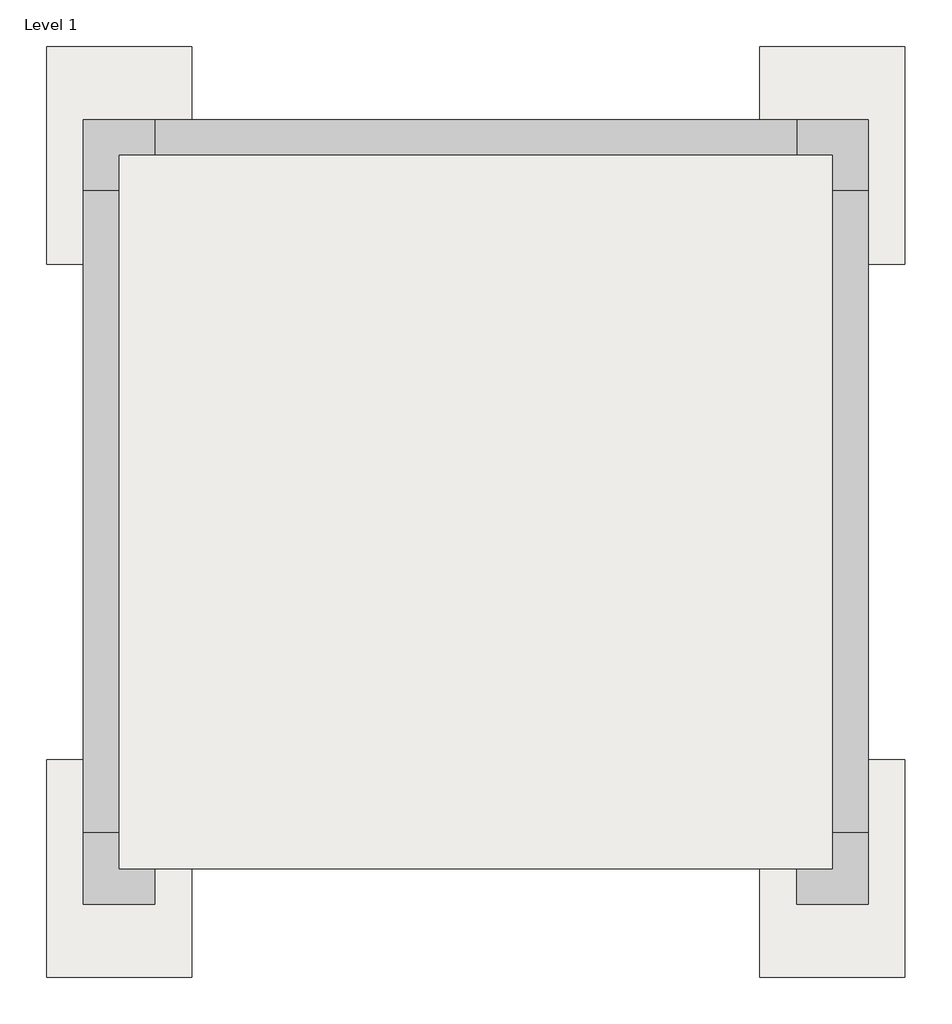
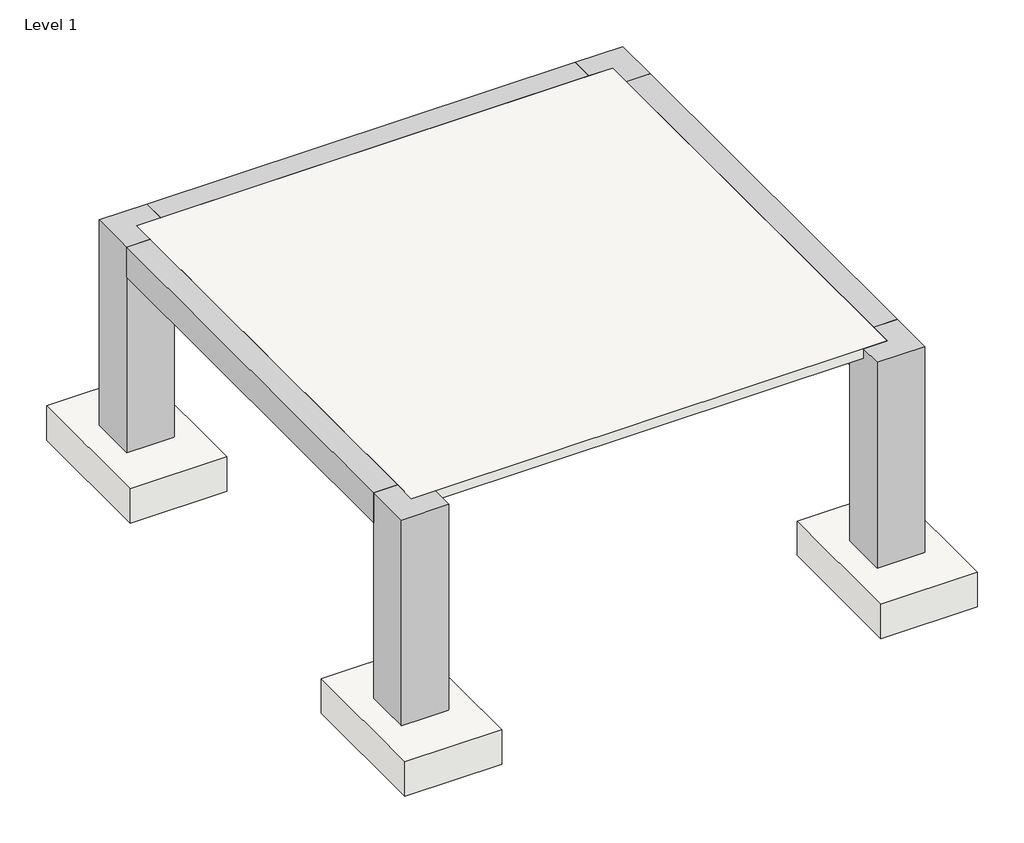
# One storey: 5 slabs, 4 columns, 3 beams.
"""IFC4 building model written with IfcOpenShell, lengths in millimetres."""

import ifcopenshell
import ifcopenshell.guid

model = None  # the IFC model being written
_history = None  # IfcOwnerHistory: only IFC2X3 demands one
_inside = {}  # id of a spatial element -> (the spatial element, [elements in it])
_under = {}  # id of a project, library or spatial element -> (it, [spatial elements below it])
_declared = {}  # id of a project -> (the project, [libraries it declares])
_typed = {}  # id of a type object -> (the type object, [elements of that type])
_made_of = {}  # id of a material, layer set ... -> (it, [elements and type objects made of it])


def new_model(schema):
    """Start an empty IFC model of exactly this schema.

    Asked for "IFC4X3", IfcOpenShell would pick the latest addendum, in which some entities
    have other attributes; the version numbers below select the first issue.
    IFC2X3 requires an IfcOwnerHistory on every rooted entity: one is made here for all.
    """
    global model, _history
    if schema == "IFC4X3":
        model = ifcopenshell.file(schema_version=(4, 3, 0, 0))
    else:
        model = ifcopenshell.file(schema=schema)
    _inside.clear()
    _under.clear()
    _declared.clear()
    _typed.clear()
    _made_of.clear()
    _history = None
    if model.schema == "IFC2X3":
        org = make("IfcOrganization", Name="unknown")
        user = make(
            "IfcPersonAndOrganization",
            ThePerson=make("IfcPerson", FamilyName="unknown"),
            TheOrganization=org,
        )
        app = make(
            "IfcApplication",
            ApplicationDeveloper=org,
            Version="unknown",
            ApplicationFullName="unknown",
            ApplicationIdentifier="unknown",
        )
        _history = make(
            "IfcOwnerHistory",
            OwningUser=user,
            OwningApplication=app,
            ChangeAction="ADDED",
            CreationDate=0,
        )
    return model


def make(cls, **values):
    """One entity of the class cls with the attributes given. An attribute that is None is left unset."""
    return model.create_entity(
        cls, **{name: value for name, value in values.items() if value is not None}
    )


def rooted(cls, **values):
    """An entity with a GlobalId (a new one), such as an element, a storey or a relation."""
    return make(cls, GlobalId=ifcopenshell.guid.new(), OwnerHistory=_history, **values)


def si_unit(unit_type, name, prefix=None):
    """IfcSIUnit, for example si_unit("LENGTHUNIT", "METRE", prefix="MILLI")."""
    return make("IfcSIUnit", UnitType=unit_type, Prefix=prefix, Name=name)


def assignment(units):
    """IfcUnitAssignment: the units of a project."""
    return None if units is None else make("IfcUnitAssignment", Units=units)


def point(xyz):
    """IfcCartesianPoint."""
    return None if xyz is None else make("IfcCartesianPoint", Coordinates=xyz)


def direction(xyz):
    """IfcDirection."""
    return None if xyz is None else make("IfcDirection", DirectionRatios=xyz)


def frame(location, z_axis=None, x_axis=None):
    """IfcAxis2Placement3D, a coordinate frame: its origin and axes. An axis left out is left unset."""
    return make(
        "IfcAxis2Placement3D",
        Location=point(location),
        Axis=direction(z_axis),
        RefDirection=direction(x_axis),
    )


def origin():
    """The frame at (0, 0, 0) with its axes left unset."""
    return frame((0.0, 0.0, 0.0))


def place(relative_to, where):
    """IfcLocalPlacement: puts the frame where relative to a parent placement (None: the world)."""
    return make(
        "IfcLocalPlacement", PlacementRelTo=relative_to, RelativePlacement=where
    )


def context(
    kind, dimensions, precision=None, world=None, true_north=None, identifier=None
):
    """IfcGeometricRepresentationContext, for example the 3D "Model" context."""
    return make(
        "IfcGeometricRepresentationContext",
        ContextIdentifier=identifier,
        ContextType=kind,
        CoordinateSpaceDimension=dimensions,
        Precision=precision,
        WorldCoordinateSystem=world,
        TrueNorth=true_north,
    )


def project(units=None, contexts=None):
    """IfcProject with its units and contexts."""
    return rooted(
        "IfcProject",
        Name="project",
        RepresentationContexts=contexts,
        UnitsInContext=assignment(units),
    )


def spatial(cls, under=None, at=None, **own):
    """A site, building, storey or space (cls), placed at a placement, below another one or the project."""
    s = rooted(cls, ObjectPlacement=at, **own)
    if under is not None:
        _under.setdefault(under.id(), (under, []))[1].append(s)
    return s


def polyline(points):
    """IfcPolyline through the points."""
    return make("IfcPolyline", Points=[point(p) for p in points])


def outline(outer, holes=None, kind="AREA"):
    """IfcArbitraryClosedProfileDef: a profile drawn as a closed curve; with holes, ...WithVoids."""
    if holes is None:
        return make("IfcArbitraryClosedProfileDef", ProfileType=kind, OuterCurve=outer)
    return make(
        "IfcArbitraryProfileDefWithVoids",
        ProfileType=kind,
        OuterCurve=outer,
        InnerCurves=holes,
    )


def extrude(swept, where, along, depth):
    """IfcExtrudedAreaSolid: the profile swept, set in the frame where, extruded along a direction by depth."""
    return make(
        "IfcExtrudedAreaSolid",
        SweptArea=swept,
        Position=where,
        ExtrudedDirection=direction(along),
        Depth=depth,
    )


def faces_of(points, faces, orient=None, outer=None):
    """IfcFace entities. A face is a list of loops; a loop is a list of indices into points, from 0.

    orient and outer hold one flag for each loop. By default every Orientation is true, the
    first loop of a face is its IfcFaceOuterBound and the others are IfcFaceBound.
    """
    made = []
    for i, loops in enumerate(faces):
        bounds = []
        for j, loop in enumerate(loops):
            is_outer = j == 0 if outer is None else outer[i][j]
            bounds.append(
                make(
                    "IfcFaceOuterBound" if is_outer else "IfcFaceBound",
                    Bound=make("IfcPolyLoop", Polygon=[points[k] for k in loop]),
                    Orientation=True if orient is None else orient[i][j],
                )
            )
        made.append(make("IfcFace", Bounds=bounds))
    return made


def faceted_brep(points, faces, orient=None, outer=None, voids=None):
    """IfcFacetedBrep: a solid bounded by flat faces; with voids (closed shells), ...WithVoids."""
    shared = [point(p) for p in points]
    hull = make("IfcClosedShell", CfsFaces=faces_of(shared, faces, orient, outer))
    if voids is None:
        return make("IfcFacetedBrep", Outer=hull)
    return make(
        "IfcFacetedBrepWithVoids",
        Outer=hull,
        Voids=[
            make(cls, CfsFaces=faces_of(shared, fs, o, b)) for cls, fs, o, b in voids
        ],
    )


def shape(context_of_items, identifier, shape_type, items):
    """IfcShapeRepresentation: the items that make up one representation, for example the "Body"."""
    return make(
        "IfcShapeRepresentation",
        ContextOfItems=context_of_items,
        RepresentationIdentifier=identifier,
        RepresentationType=shape_type,
        Items=items,
    )


def source(mapping_origin, context_of_items, identifier, shape_type, items):
    """IfcRepresentationMap: a shape defined once, which mapped items show again and again."""
    return make(
        "IfcRepresentationMap",
        MappingOrigin=mapping_origin,
        MappedRepresentation=shape(context_of_items, identifier, shape_type, items),
    )


def transform(
    local_origin,
    x_axis=None,
    y_axis=None,
    z_axis=None,
    scale=None,
    scale2=None,
    scale3=None,
    uniform=True,
):
    """IfcCartesianTransformationOperator3D, or its non-uniform kind. x_axis, y_axis, z_axis: its Axis1, 2, 3."""
    if uniform:
        return make(
            "IfcCartesianTransformationOperator3D",
            Axis1=direction(x_axis),
            Axis2=direction(y_axis),
            LocalOrigin=point(local_origin),
            Scale=scale,
            Axis3=direction(z_axis),
        )
    return make(
        "IfcCartesianTransformationOperator3DnonUniform",
        Axis1=direction(x_axis),
        Axis2=direction(y_axis),
        LocalOrigin=point(local_origin),
        Scale=scale,
        Axis3=direction(z_axis),
        Scale2=scale2,
        Scale3=scale3,
    )


def mapped(mapping_source, mapping_target):
    """IfcMappedItem: shows the shape of a source again, moved by a transform."""
    return make(
        "IfcMappedItem", MappingSource=mapping_source, MappingTarget=mapping_target
    )


def made_of(thing, what):
    """Note that an element or type object is made of a material, layer set ...; save() writes the relation."""
    if what is not None:
        _made_of.setdefault(what.id(), (what, []))[1].append(thing)
    return thing


def element(
    cls,
    number,
    at=None,
    inside=None,
    cuts=None,
    type_object=None,
    material=None,
    context=None,
    identifier="Body",
    shape_type=None,
    held_by="IfcProductDefinitionShape",
    body=None,
    shapes=None,
    **own,
):
    """One element of the class cls, such as IfcWall. Its Tag is "e" and its number.

    at: its placement. inside: the storey or other place that contains it. cuts: it is an
    opening in that element (IfcRelVoidsElement). A single representation is given by context,
    identifier, shape_type and body (its items); several are given by shapes. held_by: the class
    of the entity that holds the representations. save() writes the other relations.
    """
    e = rooted(cls, Tag="e%d" % number, ObjectPlacement=at, **own)
    if body is not None:
        shapes = [shape(context, identifier, shape_type, body)]
    if shapes is not None:
        e.Representation = make(held_by, Representations=shapes)
    if inside is not None:
        _inside.setdefault(inside.id(), (inside, []))[1].append(e)
    if cuts is not None:
        rooted(
            "IfcRelVoidsElement", RelatingBuildingElement=cuts, RelatedOpeningElement=e
        )
    if type_object is not None:
        _typed.setdefault(type_object.id(), (type_object, []))[1].append(e)
    return made_of(e, material)


def aggregate(whole, parts):
    """IfcRelAggregates: a whole, such as a stair, and the parts it consists of."""
    return rooted("IfcRelAggregates", RelatingObject=whole, RelatedObjects=parts)


def save(model, path):
    """Write the relations noted so far, then the file.

    IfcRelAggregates (storeys below a building ...), IfcRelContainedInSpatialStructure (elements
    in a storey), IfcRelDefinesByType, IfcRelAssociatesMaterial and IfcRelDeclares: one each for
    every whole, place, type object, material and project.
    """
    for whole, parts in _under.values():
        aggregate(whole, parts)
    for where, things in _inside.values():
        rooted(
            "IfcRelContainedInSpatialStructure",
            RelatedElements=things,
            RelatingStructure=where,
        )
    for kind, things in _typed.values():
        rooted("IfcRelDefinesByType", RelatedObjects=things, RelatingType=kind)
    for what, things in _made_of.values():
        rooted("IfcRelAssociatesMaterial", RelatedObjects=things, RelatingMaterial=what)
    for by, libraries in _declared.values():
        rooted("IfcRelDeclares", RelatingContext=by, RelatedDefinitions=libraries)
    model.write(path)


def slab_5ba74754(model_context):
    return source(origin(), model_context, "Body", "SweptSolid", [
        extrude(outline(polyline([(609.6, 914.4), (609.6, -914.4), (-609.6, -914.4), (-609.6, 914.4), (609.6, 914.4)])), frame((0.0, 0.0, -457.2), z_axis=(0.0, 0.0, 1.0), x_axis=(1.0, 0.0, 0.0)), (0.0, 0.0, 1.0), 457.2),
    ])


model = new_model("IFC4")

# Units and contexts
model_context = context("Model", 3, world=origin())
ifc_project = project(units=[si_unit("LENGTHUNIT", "METRE", prefix="MILLI")], contexts=[model_context])

# Site, building, storey
site = spatial("IfcSite", under=ifc_project)
building = spatial("IfcBuilding", under=site)
storey = spatial("IfcBuildingStorey", under=building, Name="Level 1", Elevation=0.0)

# Beams
placement = place(None, origin())
element("IfcBeam", 1, ObjectType="Concrete-Rectangular Beam : 60 x 40", at=placement, inside=storey, context=model_context, shape_type="SweptSolid", body=[
    extrude(outline(polyline([(2988.1334536, -400.0), (2388.1334536, -400.0), (2388.1334536, -127.0), (2688.1334536, -127.0), (2688.1334536, 0.0), (2988.1334536, 0.0), (2988.1334536, -400.0)])), frame((-17170.3561079, 0.0, 0.0), z_axis=(1.0, 0.0, 0.0), x_axis=(0.0, 1.0, 0.0)), (0.0, 0.0, 1.0), 5400.0),
])
element("IfcBeam", 2, ObjectType="Concrete-Rectangular Beam : 60 x 40", at=placement, inside=storey, context=model_context, shape_type="SweptSolid", body=[
    extrude(outline(polyline([(0.0, -17770.3561079), (-400.0, -17770.3561079), (-400.0, -17170.3561079), (-127.0, -17170.3561079), (-127.0, -17470.3561079), (0.0, -17470.3561079), (0.0, -17770.3561079)])), frame((0.0, -3011.8665464, 0.0), z_axis=(0.0, 1.0, 0.0), x_axis=(0.0, 0.0, 1.0)), (0.0, 0.0, 1.0), 5400.0),
])
element("IfcBeam", 3, ObjectType="Concrete-Rectangular Beam : 60 x 40", at=placement, inside=storey, context=model_context, shape_type="SweptSolid", body=[
    extrude(outline(polyline([(-400.0, -11770.3561079), (-400.0, -11170.3561079), (0.0, -11170.3561079), (0.0, -11470.3561079), (-127.0, -11470.3561079), (-127.0, -11770.3561079), (-400.0, -11770.3561079)])), frame((0.0, -3011.8665464, 0.0), z_axis=(0.0, 1.0, 0.0), x_axis=(0.0, 0.0, 1.0)), (0.0, 0.0, 1.0), 5400.0),
])

# Columns
element("IfcColumn", 4, ObjectType="Concrete-Rectangular-Column : 60 x 60", at=placement, inside=storey, context=model_context, shape_type="Brep", body=[
    faceted_brep([(-17170.3561079, 2988.1334536, -2743.2), (-17170.3561079, 2388.1334536, -2743.2), (-17770.3561079, 2388.1334536, -2743.2), (-17770.3561079, 2988.1334536, -2743.2), (-17170.3561079, 2988.1334536, 0.0), (-17170.3561079, 2688.1334536, 0.0), (-17170.3561079, 2688.1334536, -127.0), (-17170.3561079, 2388.1334536, -127.0), (-17470.3561079, 2388.1334536, -127.0), (-17470.3561079, 2388.1334536, 0.0), (-17770.3561079, 2388.1334536, 0.0), (-17770.3561079, 2988.1334536, 0.0), (-17470.3561079, 2688.1334536, 0.0), (-17470.3561079, 2688.1334536, -127.0)], [[[0, 1, 2, 3]], [[1, 0, 4, 5, 6, 7]], [[2, 1, 7, 8, 9, 10]], [[3, 2, 10, 11]], [[0, 3, 11, 4]], [[11, 10, 9, 12, 5, 4]], [[6, 13, 8, 7]], [[13, 12, 9, 8]], [[12, 13, 6, 5]]]),
])
element("IfcColumn", 5, ObjectType="Concrete-Rectangular-Column : 60 x 60", at=placement, inside=storey, context=model_context, shape_type="Brep", body=[
    faceted_brep([(-11170.3561079, 2988.1334536, -2743.2), (-11170.3561079, 2388.1334536, -2743.2), (-11770.3561079, 2388.1334536, -2743.2), (-11770.3561079, 2988.1334536, -2743.2), (-11170.3561079, 2988.1334536, 0.0), (-11170.3561079, 2388.1334536, 0.0), (-11470.3561079, 2388.1334536, 0.0), (-11470.3561079, 2388.1334536, -127.0), (-11770.3561079, 2388.1334536, -127.0), (-11770.3561079, 2688.1334536, -127.0), (-11770.3561079, 2688.1334536, 0.0), (-11770.3561079, 2988.1334536, 0.0), (-11470.3561079, 2688.1334536, 0.0), (-11470.3561079, 2688.1334536, -127.0)], [[[0, 1, 2, 3]], [[1, 0, 4, 5]], [[2, 1, 5, 6, 7, 8]], [[3, 2, 8, 9, 10, 11]], [[0, 3, 11, 4]], [[5, 4, 11, 10, 12, 6]], [[7, 13, 9, 8]], [[13, 12, 10, 9]], [[12, 13, 7, 6]]]),
])
element("IfcColumn", 6, ObjectType="Concrete-Rectangular-Column : 60 x 60", at=placement, inside=storey, context=model_context, shape_type="Brep", body=[
    faceted_brep([(-11170.3561079, -3011.8665464, -2743.2), (-11170.3561079, -3611.8665464, -2743.2), (-11770.3561079, -3611.8665464, -2743.2), (-11770.3561079, -3011.8665464, -2743.2), (-11170.3561079, -3011.8665464, 0.0), (-11170.3561079, -3611.8665464, 0.0), (-11770.3561079, -3611.8665464, 0.0), (-11770.3561079, -3311.8665464, 0.0), (-11770.3561079, -3311.8665464, -127.0), (-11770.3561079, -3011.8665464, -127.0), (-11470.3561079, -3011.8665464, -127.0), (-11470.3561079, -3011.8665464, 0.0), (-11470.3561079, -3311.8665464, 0.0), (-11470.3561079, -3311.8665464, -127.0)], [[[0, 1, 2, 3]], [[1, 0, 4, 5]], [[2, 1, 5, 6]], [[3, 2, 6, 7, 8, 9]], [[0, 3, 9, 10, 11, 4]], [[5, 4, 11, 12, 7, 6]], [[8, 13, 10, 9]], [[13, 12, 11, 10]], [[12, 13, 8, 7]]]),
])
element("IfcColumn", 7, ObjectType="Concrete-Rectangular-Column : 60 x 60", at=placement, inside=storey, context=model_context, shape_type="Brep", body=[
    faceted_brep([(-17170.3561079, -3011.8665464, -2743.2), (-17170.3561079, -3611.8665464, -2743.2), (-17770.3561079, -3611.8665464, -2743.2), (-17770.3561079, -3011.8665464, -2743.2), (-17170.3561079, -3011.8665464, -127.0), (-17170.3561079, -3311.8665464, -127.0), (-17170.3561079, -3311.8665464, 0.0), (-17170.3561079, -3611.8665464, 0.0), (-17770.3561079, -3611.8665464, 0.0), (-17770.3561079, -3011.8665464, 0.0), (-17470.3561079, -3011.8665464, 0.0), (-17470.3561079, -3011.8665464, -127.0), (-17470.3561079, -3311.8665464, 0.0), (-17470.3561079, -3311.8665464, -127.0)], [[[0, 1, 2, 3]], [[1, 0, 4, 5, 6, 7]], [[2, 1, 7, 8]], [[3, 2, 8, 9]], [[0, 3, 9, 10, 11, 4]], [[8, 7, 6, 12, 10, 9]], [[13, 5, 4, 11]], [[12, 13, 11, 10]], [[13, 12, 6, 5]]]),
])

# Slabs
element("IfcSlab", 8, ObjectType="3\" LW Concrete on 2\" Metal Deck", at=placement, inside=storey, context=model_context, shape_type="Brep", body=[
    faceted_brep([(-17470.3561079, -3311.8665464, -127.0), (-17470.3561079, -3011.8665464, -127.0), (-17470.3561079, 2388.1334536, -127.0), (-17470.3561079, 2688.1334536, -127.0), (-17170.3561079, 2688.1334536, -127.0), (-11770.3561079, 2688.1334536, -127.0), (-11470.3561079, 2688.1334536, -127.0), (-11470.3561079, 2388.1334536, -127.0), (-11470.3561079, -3011.8665464, -127.0), (-11470.3561079, -3311.8665464, -127.0), (-11770.3561079, -3311.8665464, -127.0), (-17170.3561079, -3311.8665464, -127.0), (-17470.3561079, -3311.8665464, 0.0), (-17170.3561079, -3311.8665464, 0.0), (-11770.3561079, -3311.8665464, 0.0), (-11470.3561079, -3311.8665464, 0.0), (-11470.3561079, -3011.8665464, 0.0), (-11470.3561079, 2388.1334536, 0.0), (-11470.3561079, 2688.1334536, 0.0), (-11770.3561079, 2688.1334536, 0.0), (-17170.3561079, 2688.1334536, 0.0), (-17470.3561079, 2688.1334536, 0.0), (-17470.3561079, 2388.1334536, 0.0), (-17470.3561079, -3011.8665464, 0.0)], [[[0, 1, 2, 3, 4, 5, 6, 7, 8, 9, 10, 11]], [[12, 13, 14, 15, 16, 17, 18, 19, 20, 21, 22, 23]], [[3, 2, 1, 0, 12, 23, 22, 21]], [[6, 5, 4, 3, 21, 20, 19, 18]], [[9, 8, 7, 6, 18, 17, 16, 15]], [[0, 11, 10, 9, 15, 14, 13, 12]]]),
])
slab_shape = slab_5ba74754(model_context)
element("IfcSlab", 9, ObjectType="Footing-Rectangular : 72\" x 48\" x 18\"", at=placement, inside=storey, context=model_context, shape_type="MappedRepresentation", body=[
    mapped(slab_shape, transform((-17470.3561079, 2688.1334536, -2743.2), x_axis=(1.0, 0.0, 0.0), y_axis=(0.0, 1.0, 0.0), z_axis=(0.0, 0.0, 1.0))),
])
element("IfcSlab", 10, ObjectType="Footing-Rectangular : 72\" x 48\" x 18\"", at=placement, inside=storey, context=model_context, shape_type="MappedRepresentation", body=[
    mapped(slab_shape, transform((-11470.3561079, 2688.1334536, -2743.2), x_axis=(1.0, 0.0, 0.0), y_axis=(0.0, 1.0, 0.0), z_axis=(0.0, 0.0, 1.0))),
])
element("IfcSlab", 11, ObjectType="Footing-Rectangular : 72\" x 48\" x 18\"", at=placement, inside=storey, context=model_context, shape_type="MappedRepresentation", body=[
    mapped(slab_shape, transform((-11470.3561079, -3311.8665464, -2743.2), x_axis=(1.0, 0.0, 0.0), y_axis=(0.0, 1.0, 0.0), z_axis=(0.0, 0.0, 1.0))),
])
element("IfcSlab", 12, ObjectType="Footing-Rectangular : 72\" x 48\" x 18\"", at=placement, inside=storey, context=model_context, shape_type="MappedRepresentation", body=[
    mapped(slab_shape, transform((-17470.3561079, -3311.8665464, -2743.2), x_axis=(1.0, 0.0, 0.0), y_axis=(0.0, 1.0, 0.0), z_axis=(0.0, 0.0, 1.0))),
])

save(model, "model.ifc")

# Revit data of these elements
# Project information
#   Project Issue Date = "Issue Date"
#   Project Status = "Project Status"
#   Client Name = "Owner"
#   Project Address = "Enter address here"
#   Project Name = "Project Name"
#   Project Number = "Project Number"
# Grids (mm)
#   "1": line (4751.493, -3311.867) -> (-19494.984, -3311.867)
#   "2": line (4751.493, 2688.133) -> (-19494.984, 2688.133)
#   "3": line (4751.493, 8688.133) -> (-19494.984, 8688.133)
#   "4": line (4751.493, 14688.133) -> (-19494.984, 14688.133)
#   "A": line (-17470.356, -6595.728) -> (-17470.356, 17410.58)
#   "B": line (-11470.356, -6595.728) -> (-11470.356, 17410.58)
#   "C": line (-5470.356, -6595.728) -> (-5470.356, 17410.58)
#   "D": line (529.644, -6595.728) -> (529.644, 17410.58)
# Type "Concrete-Rectangular Beam : 60 x 40"
#   Assembly Code = "B10"
#   Length [instance default] = 1524 mm
#   b = 600 mm
#   h = 400 mm
#   Structural Material [instance default] = Concrete, Cast-in-Place gray
# Type "Concrete-Rectangular-Column : 60 x 60"
#   Assembly Code = "B10"
#   b = 600 mm
#   h = 600 mm
#   Structural Material [instance default] = Concrete, Cast-in-Place gray
# Type "3\" LW Concrete on 2\" Metal Deck"
#   Assembly Code = "B1010"
#   Thickness = 127 mm
#   Function = 0
#   Layers, outside or top first: 127 mm "Concrete, Lightweight - 4 ksi" (function 1); 0 mm "Metal Deck" (function 200)
# Type "Footing-Rectangular : 72\" x 48\" x 18\""
#   Assembly Code = "A1010100"
#   Width = 1219.2 mm
#   Length = 1828.8 mm
#   Thickness = 457.2 mm
#   Structural Material [instance default] = Concrete, Cast-in-Place gray
# Element 1 (IfcBeam, "Concrete-Rectangular Beam : 60 x 40")
#   Comments = ""
#   Structural Material = Concrete, Cast-in-Place gray
#   Phase Created = New Construction
#   Materials on its faces: "Concrete, Cast-in-Place gray"
# Elements 2, 3 (IfcBeam, "Concrete-Rectangular Beam : 60 x 40")
#   Comments = ""
#   Structural Material = Concrete, Cast-in-Place gray
#   Phase Created = New Construction
#   Materials on its faces: "Concrete, Cast-in-Place gray", "Metal Deck"
# Elements 4, 5, 6, 7 (IfcColumn, "Concrete-Rectangular-Column : 60 x 60")
#   Comments = ""
#   Structural Material = Concrete, Cast-in-Place gray
#   Phase Created = New Construction
#   Materials on its faces: "Concrete, Cast-in-Place gray"
# Element 8 (IfcSlab, "3\" LW Concrete on 2\" Metal Deck")
#   built-in parameter 1001955 = -1.5708 (stored number, unit not read)
#   Height Offset From Level = 0 mm
#   built-in parameter 1001954 = 1
#   Phase Created = New Construction
#   Materials on its faces: "Metal Deck", "Concrete, Lightweight - 4 ksi"
# Elements 9, 10, 11, 12 (IfcSlab, "Footing-Rectangular : 72\" x 48\" x 18\"")
#   Structural Material = Concrete, Cast-in-Place gray
#   Phase Created = New Construction
#   Materials on its faces: "Concrete, Cast-in-Place gray"
# Materials
#   "Concrete, Cast-in-Place gray": class "Concrete", colour RGB 192 192 192, transparency 0, Description = "Cast-in-place concrete", Cost = 0
#   "Concrete, Lightweight - 4 ksi": class "Concrete", colour RGB 127 127 127, transparency 0, Description = "Lightweight concrete 4 ksi", Cost = 0
#   "Metal Deck": class "Metal", colour RGB 199 199 199, transparency 0, Description = "Steel, mill finish", Cost = 0
